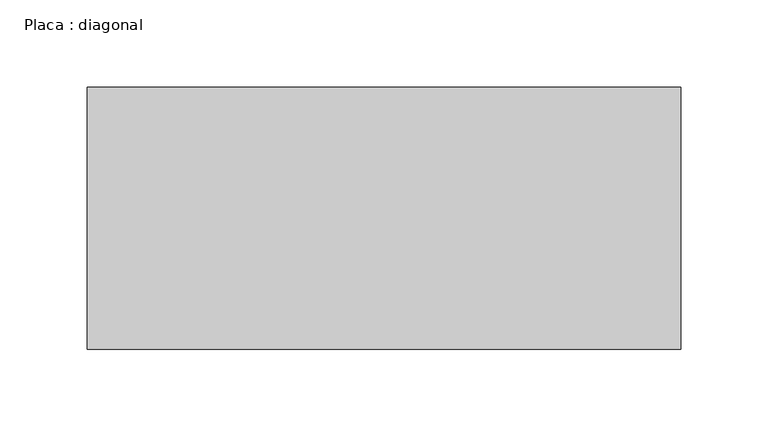
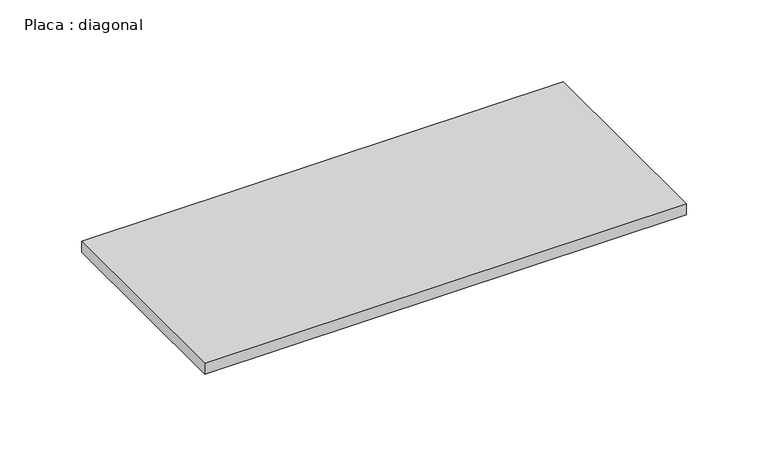
"""IFC4 building model written with IfcOpenShell, lengths in millimetres: beam geometry, Placa : diagonal."""

from ifc_helpers import new_model, si_unit, frame, origin, place, context, project, spatial, polyline, outline, extrude, source, transform, mapped, element, save


def placa_diagonal_1af65b22(model_context):
    return source(origin(), model_context, "Body", "SweptSolid", [
        extrude(outline(polyline([(169.9719585, 75.0), (169.9719585, -75.0), (-169.5739238, -75.0), (-169.5739238, 75.0), (169.9719585, 75.0)])), frame((0.0, 0.0, -4.0), z_axis=(0.0, 0.0, 1.0), x_axis=(1.0, 0.0, 0.0)), (0.0, 0.0, 1.0), 8.0),
    ])


if __name__ == "__main__":
    model = new_model("IFC4")
    model_context = context("Model", 3, world=origin())
    ifc_project = project(units=[si_unit("LENGTHUNIT", "METRE", prefix="MILLI")], contexts=[model_context])
    site = spatial("IfcSite", under=ifc_project)
    building = spatial("IfcBuilding", under=site)
    placement = place(None, origin())
    placa_diagonal_shape = placa_diagonal_1af65b22(model_context)
    element("IfcBeam", 1, ObjectType="Placa : diagonal", at=placement, inside=building, context=model_context, shape_type="MappedRepresentation", body=[
        mapped(placa_diagonal_shape, transform((0.0, 0.0, 0.0), x_axis=(1.0, 0.0, 0.0), y_axis=(0.0, 1.0, 0.0), z_axis=(0.0, 0.0, 1.0))),
    ])
    save(model, "model.ifc")

# Revit data of these elements
# Type "Placa : diagonal"
#   W = 0
#   Length [instance default] = 1.50 m
#   b = 0.15 m
#   d = 0.008 m
#   A = 0 m²
#   Structural Material [instance default] = Aço, 45-345
# Element 1 (IfcBeam, "Placa : diagonal")
#   Materials on its faces: "Aço, 45-345"
# Materials
#   "Aço, 45-345": class "Metal", colour RGB 247 247 247, transparency 0, Description = "Aço 345 MPa", Cost = 0
